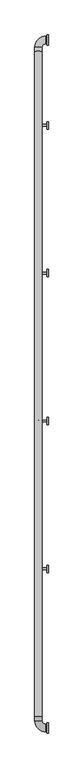
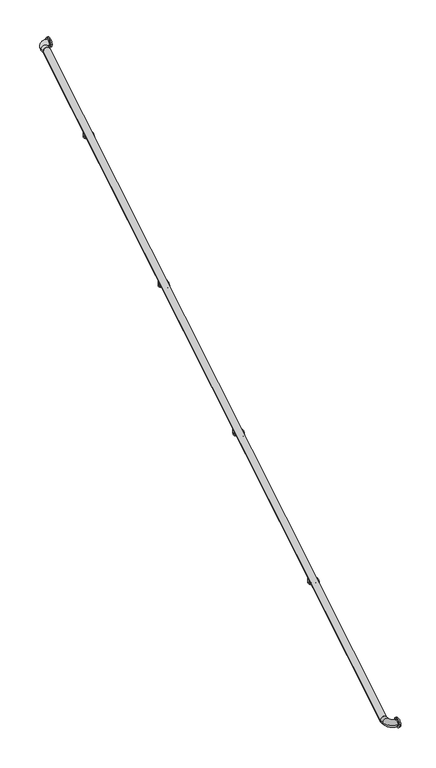
"""IFC4 building model written with IfcOpenShell, lengths in millimetres: railing geometry."""

from ifc_helpers import new_model, si_unit, point, frame, frame_2d, origin, place, context, project, spatial, circle_curve, ellipse_curve, trimmed, segment, composite_curve, outline, extrude, source, transform, mapped, element, save
from ifc_brep_helpers import plane_surface, cylinder_surface, revolved_surface, advanced_brep


def railing_debc8759(model_context):
    return source(origin(), model_context, "Body", "SolidModel", [
        advanced_brep(
        [(20407.2944438, 42249.3496945, 1051.653859), (20458.0944438, 42249.3496945, 1051.653859), (20407.2944438, 46749.3496945, 3771.653859), (20458.0944438, 46749.3496945, 3771.653859)],
        [
            (0, 1, ellipse_curve(frame((20432.6944438, 42249.3496945, 1051.653859), z_axis=(0.0, -1.0, 0.0), x_axis=(0.0, 0.0, -1.0)), 29.6794743, 25.4)),
            (1, 0, ellipse_curve(frame((20432.6944438, 42249.3496945, 1051.653859), z_axis=(0.0, -1.0, 0.0), x_axis=(0.0, 0.0, -1.0)), 29.6794743, 25.4)),
            (2, 3, ellipse_curve(frame((20432.6944438, 46749.3496945, 3771.653859), z_axis=(0.0, 1.0, 0.0), x_axis=(0.0, 0.0, -1.0)), 29.6794743, 25.4)),
            (3, 2, ellipse_curve(frame((20432.6944438, 46749.3496945, 3771.653859), z_axis=(0.0, 1.0, 0.0), x_axis=(0.0, 0.0, -1.0)), 29.6794743, 25.4)),
            (0, 2),
            (3, 1),
        ],
        [
            plane_surface(frame((20432.6944438, 42249.3496945, 1081.3333333), z_axis=(0.0, -1.0, 0.0), x_axis=(0.0, 0.0, 1.0))),
            plane_surface(frame((20432.6944438, 46749.3496945, 3801.3333333), z_axis=(0.0, 1.0, 0.0), x_axis=(0.0, 0.0, 1.0))),
            cylinder_surface(frame((20432.6944438, 42262.4888551, 1059.5957516), z_axis=(0.0, -0.8558103053667958, -0.5172897845772637), x_axis=(1.0, 0.0, 0.0)), 25.4),
        ],
        [
            (0, [[1, 2]]),
            (1, [[3, 4]]),
            (2, [[-1, 5, -4, 6]]),
            (2, [[-2, -6, -3, -5]]),
        ],
    ),
        extrude(outline(composite_curve([segment(trimmed(circle_curve(frame_2d((46249.3496945, 3363.7521624)), 25.4), [point((46274.7496945, 3363.7521624))], [point((46223.9496945, 3363.7521624))], False, "CARTESIAN"), True, "CONTINUOUS"), segment(trimmed(circle_curve(frame_2d((46249.3496945, 3363.7521624)), 25.4), [point((46223.9496945, 3363.7521624))], [point((46274.7496945, 3363.7521624))], False, "CARTESIAN"), True, "CONTINUOUS")], self_intersect=False)), frame((20490.1194438, 0.0, 0.0), z_axis=(1.0, 0.0, 0.0), x_axis=(0.0, 1.0, 0.0)), (0.0, 0.0, 1.0), 9.525),
        advanced_brep(
        [(20432.6444438, 46242.9996945, 3439.7521624), (20432.6444438, 46255.6996945, 3439.7521624), (20432.6444438, 46242.9996945, 3382.8021624), (20432.6444438, 46255.6996945, 3382.8021624), (20451.6944438, 46255.6996945, 3363.7521624), (20451.6944438, 46242.9996945, 3363.7521624), (20490.1194438, 46242.9996945, 3363.7521624), (20490.1194438, 46255.6996945, 3363.7521624)],
        [
            (0, 1, circle_curve(frame((20432.6444438, 46249.3496945, 3439.7521624), z_axis=(0.0, 0.0, 1.0), x_axis=(0.0, 1.0, 0.0)), 6.35)),
            (1, 0, circle_curve(frame((20432.6444438, 46249.3496945, 3439.7521624), z_axis=(0.0, 0.0, 1.0), x_axis=(0.0, 1.0, 0.0)), 6.35)),
            (0, 2),
            (2, 3, circle_curve(frame((20432.6444438, 46249.3496945, 3382.8021624), z_axis=(0.0, 0.0, 1.0), x_axis=(0.0, 1.0, 0.0)), 6.35)),
            (3, 1),
            (3, 2, circle_curve(frame((20432.6444438, 46249.3496945, 3382.8021624), z_axis=(0.0, 0.0, 1.0), x_axis=(0.0, 1.0, 0.0)), 6.35)),
            (4, 3, circle_curve(frame((20451.6944438, 46255.6996945, 3382.8021624), z_axis=(0.0, 1.0, 0.0), x_axis=(-1.0, 0.0, 0.0)), 19.05)),
            (2, 5, circle_curve(frame((20451.6944438, 46242.9996945, 3382.8021624), z_axis=(0.0, -1.0, 0.0), x_axis=(-1.0, 0.0, 0.0)), 19.05)),
            (5, 4, circle_curve(frame((20451.6944438, 46249.3496945, 3363.7521624), z_axis=(-1.0, 0.0, 0.0), x_axis=(0.0, 1.0, 0.0)), 6.35)),
            (4, 5, circle_curve(frame((20451.6944438, 46249.3496945, 3363.7521624), z_axis=(-1.0, 0.0, 0.0), x_axis=(0.0, 1.0, 0.0)), 6.35)),
            (6, 7, circle_curve(frame((20490.1194438, 46249.3496945, 3363.7521624), z_axis=(1.0, 0.0, 0.0), x_axis=(0.0, 1.0, 0.0)), 6.35)),
            (7, 6, circle_curve(frame((20490.1194438, 46249.3496945, 3363.7521624), z_axis=(1.0, 0.0, 0.0), x_axis=(0.0, 1.0, 0.0)), 6.35)),
            (5, 6),
            (7, 4),
        ],
        [
            plane_surface(frame((20432.6444438, 46255.6996945, 3439.7521624), z_axis=(0.0, 0.0, 1.0), x_axis=(1.0, 0.0, 0.0))),
            cylinder_surface(frame((20432.6444438, 46249.3496945, 3439.7521624), z_axis=(0.0, 0.0, 1.0), x_axis=(0.0, 1.0, 0.0)), 6.35),
            revolved_surface(trimmed(ellipse_curve(frame((20432.6444438, 46249.3496945, 3382.8021624), z_axis=(0.0, 0.0, 1.0), x_axis=(0.0, 1.0, 0.0)), 6.35, 6.35), [point((20432.6444438, 46242.9996945, 3382.8021624))], [point((20432.6444438, 46255.6996945, 3382.8021624))], True, "CARTESIAN"), (20451.6944438, 46249.3496945, 3382.8021624), (0.0, -1.0, 0.0)),
            revolved_surface(trimmed(ellipse_curve(frame((20432.6444438, 46249.3496945, 3382.8021624), z_axis=(0.0, 0.0, 1.0), x_axis=(0.0, 1.0, 0.0)), 6.35, 6.35), [point((20432.6444438, 46255.6996945, 3382.8021624))], [point((20432.6444438, 46242.9996945, 3382.8021624))], True, "CARTESIAN"), (20451.6944438, 46249.3496945, 3382.8021624), (0.0, -1.0, 0.0)),
            plane_surface(frame((20490.1194438, 46249.3496945, 3357.4021624), z_axis=(1.0, 0.0, 0.0), x_axis=(0.0, 1.0, 0.0))),
            cylinder_surface(frame((20451.6944438, 46249.3496945, 3363.7521624), z_axis=(-1.0, 0.0, 0.0), x_axis=(0.0, 1.0, 0.0)), 6.35),
        ],
        [
            (0, [[1, 2]]),
            (1, [[-1, 3, 4, 5]]),
            (1, [[-2, -5, 6, -3]]),
            (2, [[7, -4, 8, 9]]),
            (3, [[-8, -6, -7, 10]]),
            (4, [[11, 12]]),
            (5, [[-9, 13, -12, 14]]),
            (5, [[-10, -14, -11, -13]]),
        ],
    ),
        extrude(outline(composite_curve([segment(trimmed(circle_curve(frame_2d((45249.3496945, 2759.307718)), 25.4), [point((45274.7496945, 2759.307718))], [point((45223.9496945, 2759.307718))], False, "CARTESIAN"), True, "CONTINUOUS"), segment(trimmed(circle_curve(frame_2d((45249.3496945, 2759.307718)), 25.4), [point((45223.9496945, 2759.307718))], [point((45274.7496945, 2759.307718))], False, "CARTESIAN"), True, "CONTINUOUS")], self_intersect=False)), frame((20490.1194438, 0.0, 0.0), z_axis=(1.0, 0.0, 0.0), x_axis=(0.0, 1.0, 0.0)), (0.0, 0.0, 1.0), 9.525),
        advanced_brep(
        [(20432.6444438, 45242.9996945, 2835.307718), (20432.6444438, 45255.6996945, 2835.307718), (20432.6444438, 45242.9996945, 2778.357718), (20432.6444438, 45255.6996945, 2778.357718), (20451.6944438, 45255.6996945, 2759.307718), (20451.6944438, 45242.9996945, 2759.307718), (20490.1194438, 45242.9996945, 2759.307718), (20490.1194438, 45255.6996945, 2759.307718)],
        [
            (0, 1, circle_curve(frame((20432.6444438, 45249.3496945, 2835.307718), z_axis=(0.0, 0.0, 1.0), x_axis=(0.0, 1.0, 0.0)), 6.35)),
            (1, 0, circle_curve(frame((20432.6444438, 45249.3496945, 2835.307718), z_axis=(0.0, 0.0, 1.0), x_axis=(0.0, 1.0, 0.0)), 6.35)),
            (0, 2),
            (2, 3, circle_curve(frame((20432.6444438, 45249.3496945, 2778.357718), z_axis=(0.0, 0.0, 1.0), x_axis=(0.0, 1.0, 0.0)), 6.35)),
            (3, 1),
            (3, 2, circle_curve(frame((20432.6444438, 45249.3496945, 2778.357718), z_axis=(0.0, 0.0, 1.0), x_axis=(0.0, 1.0, 0.0)), 6.35)),
            (4, 3, circle_curve(frame((20451.6944438, 45255.6996945, 2778.357718), z_axis=(0.0, 1.0, 0.0), x_axis=(-1.0, 0.0, 0.0)), 19.05)),
            (2, 5, circle_curve(frame((20451.6944438, 45242.9996945, 2778.357718), z_axis=(0.0, -1.0, 0.0), x_axis=(-1.0, 0.0, 0.0)), 19.05)),
            (5, 4, circle_curve(frame((20451.6944438, 45249.3496945, 2759.307718), z_axis=(-1.0, 0.0, 0.0), x_axis=(0.0, 1.0, 0.0)), 6.35)),
            (4, 5, circle_curve(frame((20451.6944438, 45249.3496945, 2759.307718), z_axis=(-1.0, 0.0, 0.0), x_axis=(0.0, 1.0, 0.0)), 6.35)),
            (6, 7, circle_curve(frame((20490.1194438, 45249.3496945, 2759.307718), z_axis=(1.0, 0.0, 0.0), x_axis=(0.0, 1.0, 0.0)), 6.35)),
            (7, 6, circle_curve(frame((20490.1194438, 45249.3496945, 2759.307718), z_axis=(1.0, 0.0, 0.0), x_axis=(0.0, 1.0, 0.0)), 6.35)),
            (5, 6),
            (7, 4),
        ],
        [
            plane_surface(frame((20432.6444438, 45255.6996945, 2835.307718), z_axis=(0.0, 0.0, 1.0), x_axis=(1.0, 0.0, 0.0))),
            cylinder_surface(frame((20432.6444438, 45249.3496945, 2835.307718), z_axis=(0.0, 0.0, 1.0), x_axis=(0.0, 1.0, 0.0)), 6.35),
            revolved_surface(trimmed(ellipse_curve(frame((20432.6444438, 45249.3496945, 2778.357718), z_axis=(0.0, 0.0, 1.0), x_axis=(0.0, 1.0, 0.0)), 6.35, 6.35), [point((20432.6444438, 45242.9996945, 2778.357718))], [point((20432.6444438, 45255.6996945, 2778.357718))], True, "CARTESIAN"), (20451.6944438, 45249.3496945, 2778.357718), (0.0, -1.0, 0.0)),
            revolved_surface(trimmed(ellipse_curve(frame((20432.6444438, 45249.3496945, 2778.357718), z_axis=(0.0, 0.0, 1.0), x_axis=(0.0, 1.0, 0.0)), 6.35, 6.35), [point((20432.6444438, 45255.6996945, 2778.357718))], [point((20432.6444438, 45242.9996945, 2778.357718))], True, "CARTESIAN"), (20451.6944438, 45249.3496945, 2778.357718), (0.0, -1.0, 0.0)),
            plane_surface(frame((20490.1194438, 45249.3496945, 2752.957718), z_axis=(1.0, 0.0, 0.0), x_axis=(0.0, 1.0, 0.0))),
            cylinder_surface(frame((20451.6944438, 45249.3496945, 2759.307718), z_axis=(-1.0, 0.0, 0.0), x_axis=(0.0, 1.0, 0.0)), 6.35),
        ],
        [
            (0, [[1, 2]]),
            (1, [[-1, 3, 4, 5]]),
            (1, [[-2, -5, 6, -3]]),
            (2, [[7, -4, 8, 9]]),
            (3, [[-8, -6, -7, 10]]),
            (4, [[11, 12]]),
            (5, [[-9, 13, -12, 14]]),
            (5, [[-10, -14, -11, -13]]),
        ],
    ),
        extrude(outline(composite_curve([segment(trimmed(circle_curve(frame_2d((44249.3496945, 2154.8632735)), 25.4), [point((44274.7496945, 2154.8632735))], [point((44223.9496945, 2154.8632735))], False, "CARTESIAN"), True, "CONTINUOUS"), segment(trimmed(circle_curve(frame_2d((44249.3496945, 2154.8632735)), 25.4), [point((44223.9496945, 2154.8632735))], [point((44274.7496945, 2154.8632735))], False, "CARTESIAN"), True, "CONTINUOUS")], self_intersect=False)), frame((20490.1194438, 0.0, 0.0), z_axis=(1.0, 0.0, 0.0), x_axis=(0.0, 1.0, 0.0)), (0.0, 0.0, 1.0), 9.525),
        advanced_brep(
        [(20432.6444438, 44242.9996945, 2230.8632735), (20432.6444438, 44255.6996945, 2230.8632735), (20432.6444438, 44242.9996945, 2173.9132735), (20432.6444438, 44255.6996945, 2173.9132735), (20451.6944438, 44255.6996945, 2154.8632735), (20451.6944438, 44242.9996945, 2154.8632735), (20490.1194438, 44242.9996945, 2154.8632735), (20490.1194438, 44255.6996945, 2154.8632735)],
        [
            (0, 1, circle_curve(frame((20432.6444438, 44249.3496945, 2230.8632735), z_axis=(0.0, 0.0, 1.0), x_axis=(0.0, 1.0, 0.0)), 6.35)),
            (1, 0, circle_curve(frame((20432.6444438, 44249.3496945, 2230.8632735), z_axis=(0.0, 0.0, 1.0), x_axis=(0.0, 1.0, 0.0)), 6.35)),
            (0, 2),
            (2, 3, circle_curve(frame((20432.6444438, 44249.3496945, 2173.9132735), z_axis=(0.0, 0.0, 1.0), x_axis=(0.0, 1.0, 0.0)), 6.35)),
            (3, 1),
            (3, 2, circle_curve(frame((20432.6444438, 44249.3496945, 2173.9132735), z_axis=(0.0, 0.0, 1.0), x_axis=(0.0, 1.0, 0.0)), 6.35)),
            (4, 3, circle_curve(frame((20451.6944438, 44255.6996945, 2173.9132735), z_axis=(0.0, 1.0, 0.0), x_axis=(-1.0, 0.0, 0.0)), 19.05)),
            (2, 5, circle_curve(frame((20451.6944438, 44242.9996945, 2173.9132735), z_axis=(0.0, -1.0, 0.0), x_axis=(-1.0, 0.0, 0.0)), 19.05)),
            (5, 4, circle_curve(frame((20451.6944438, 44249.3496945, 2154.8632735), z_axis=(-1.0, 0.0, 0.0), x_axis=(0.0, 1.0, 0.0)), 6.35)),
            (4, 5, circle_curve(frame((20451.6944438, 44249.3496945, 2154.8632735), z_axis=(-1.0, 0.0, 0.0), x_axis=(0.0, 1.0, 0.0)), 6.35)),
            (6, 7, circle_curve(frame((20490.1194438, 44249.3496945, 2154.8632735), z_axis=(1.0, 0.0, 0.0), x_axis=(0.0, 1.0, 0.0)), 6.35)),
            (7, 6, circle_curve(frame((20490.1194438, 44249.3496945, 2154.8632735), z_axis=(1.0, 0.0, 0.0), x_axis=(0.0, 1.0, 0.0)), 6.35)),
            (5, 6),
            (7, 4),
        ],
        [
            plane_surface(frame((20432.6444438, 44255.6996945, 2230.8632735), z_axis=(0.0, 0.0, 1.0), x_axis=(1.0, 0.0, 0.0))),
            cylinder_surface(frame((20432.6444438, 44249.3496945, 2230.8632735), z_axis=(0.0, 0.0, 1.0), x_axis=(0.0, 1.0, 0.0)), 6.35),
            revolved_surface(trimmed(ellipse_curve(frame((20432.6444438, 44249.3496945, 2173.9132735), z_axis=(0.0, 0.0, 1.0), x_axis=(0.0, 1.0, 0.0)), 6.35, 6.35), [point((20432.6444438, 44242.9996945, 2173.9132735))], [point((20432.6444438, 44255.6996945, 2173.9132735))], True, "CARTESIAN"), (20451.6944438, 44249.3496945, 2173.9132735), (0.0, -1.0, 0.0)),
            revolved_surface(trimmed(ellipse_curve(frame((20432.6444438, 44249.3496945, 2173.9132735), z_axis=(0.0, 0.0, 1.0), x_axis=(0.0, 1.0, 0.0)), 6.35, 6.35), [point((20432.6444438, 44255.6996945, 2173.9132735))], [point((20432.6444438, 44242.9996945, 2173.9132735))], True, "CARTESIAN"), (20451.6944438, 44249.3496945, 2173.9132735), (0.0, -1.0, 0.0)),
            plane_surface(frame((20490.1194438, 44249.3496945, 2148.5132735), z_axis=(1.0, 0.0, 0.0), x_axis=(0.0, 1.0, 0.0))),
            cylinder_surface(frame((20451.6944438, 44249.3496945, 2154.8632735), z_axis=(-1.0, 0.0, 0.0), x_axis=(0.0, 1.0, 0.0)), 6.35),
        ],
        [
            (0, [[1, 2]]),
            (1, [[-1, 3, 4, 5]]),
            (1, [[-2, -5, 6, -3]]),
            (2, [[7, -4, 8, 9]]),
            (3, [[-8, -6, -7, 10]]),
            (4, [[11, 12]]),
            (5, [[-9, 13, -12, 14]]),
            (5, [[-10, -14, -11, -13]]),
        ],
    ),
        extrude(outline(composite_curve([segment(trimmed(circle_curve(frame_2d((43249.3496945, 1550.4188291)), 25.4), [point((43274.7496945, 1550.4188291))], [point((43223.9496945, 1550.4188291))], False, "CARTESIAN"), True, "CONTINUOUS"), segment(trimmed(circle_curve(frame_2d((43249.3496945, 1550.4188291)), 25.4), [point((43223.9496945, 1550.4188291))], [point((43274.7496945, 1550.4188291))], False, "CARTESIAN"), True, "CONTINUOUS")], self_intersect=False)), frame((20490.1194438, 0.0, 0.0), z_axis=(1.0, 0.0, 0.0), x_axis=(0.0, 1.0, 0.0)), (0.0, 0.0, 1.0), 9.525),
        advanced_brep(
        [(20432.6444438, 43242.9996945, 1626.4188291), (20432.6444438, 43255.6996945, 1626.4188291), (20432.6444438, 43242.9996945, 1569.4688291), (20432.6444438, 43255.6996945, 1569.4688291), (20451.6944438, 43255.6996945, 1550.4188291), (20451.6944438, 43242.9996945, 1550.4188291), (20490.1194438, 43242.9996945, 1550.4188291), (20490.1194438, 43255.6996945, 1550.4188291)],
        [
            (0, 1, circle_curve(frame((20432.6444438, 43249.3496945, 1626.4188291), z_axis=(0.0, 0.0, 1.0), x_axis=(0.0, 1.0, 0.0)), 6.35)),
            (1, 0, circle_curve(frame((20432.6444438, 43249.3496945, 1626.4188291), z_axis=(0.0, 0.0, 1.0), x_axis=(0.0, 1.0, 0.0)), 6.35)),
            (0, 2),
            (2, 3, circle_curve(frame((20432.6444438, 43249.3496945, 1569.4688291), z_axis=(0.0, 0.0, 1.0), x_axis=(0.0, 1.0, 0.0)), 6.35)),
            (3, 1),
            (3, 2, circle_curve(frame((20432.6444438, 43249.3496945, 1569.4688291), z_axis=(0.0, 0.0, 1.0), x_axis=(0.0, 1.0, 0.0)), 6.35)),
            (4, 3, circle_curve(frame((20451.6944438, 43255.6996945, 1569.4688291), z_axis=(0.0, 1.0, 0.0), x_axis=(-1.0, 0.0, 0.0)), 19.05)),
            (2, 5, circle_curve(frame((20451.6944438, 43242.9996945, 1569.4688291), z_axis=(0.0, -1.0, 0.0), x_axis=(-1.0, 0.0, 0.0)), 19.05)),
            (5, 4, circle_curve(frame((20451.6944438, 43249.3496945, 1550.4188291), z_axis=(-1.0, 0.0, 0.0), x_axis=(0.0, 1.0, 0.0)), 6.35)),
            (4, 5, circle_curve(frame((20451.6944438, 43249.3496945, 1550.4188291), z_axis=(-1.0, 0.0, 0.0), x_axis=(0.0, 1.0, 0.0)), 6.35)),
            (6, 7, circle_curve(frame((20490.1194438, 43249.3496945, 1550.4188291), z_axis=(1.0, 0.0, 0.0), x_axis=(0.0, 1.0, 0.0)), 6.35)),
            (7, 6, circle_curve(frame((20490.1194438, 43249.3496945, 1550.4188291), z_axis=(1.0, 0.0, 0.0), x_axis=(0.0, 1.0, 0.0)), 6.35)),
            (5, 6),
            (7, 4),
        ],
        [
            plane_surface(frame((20432.6444438, 43255.6996945, 1626.4188291), z_axis=(0.0, 0.0, 1.0), x_axis=(1.0, 0.0, 0.0))),
            cylinder_surface(frame((20432.6444438, 43249.3496945, 1626.4188291), z_axis=(0.0, 0.0, 1.0), x_axis=(0.0, 1.0, 0.0)), 6.35),
            revolved_surface(trimmed(ellipse_curve(frame((20432.6444438, 43249.3496945, 1569.4688291), z_axis=(0.0, 0.0, 1.0), x_axis=(0.0, 1.0, 0.0)), 6.35, 6.35), [point((20432.6444438, 43242.9996945, 1569.4688291))], [point((20432.6444438, 43255.6996945, 1569.4688291))], True, "CARTESIAN"), (20451.6944438, 43249.3496945, 1569.4688291), (0.0, -1.0, 0.0)),
            revolved_surface(trimmed(ellipse_curve(frame((20432.6444438, 43249.3496945, 1569.4688291), z_axis=(0.0, 0.0, 1.0), x_axis=(0.0, 1.0, 0.0)), 6.35, 6.35), [point((20432.6444438, 43255.6996945, 1569.4688291))], [point((20432.6444438, 43242.9996945, 1569.4688291))], True, "CARTESIAN"), (20451.6944438, 43249.3496945, 1569.4688291), (0.0, -1.0, 0.0)),
            plane_surface(frame((20490.1194438, 43249.3496945, 1544.0688291), z_axis=(1.0, 0.0, 0.0), x_axis=(0.0, 1.0, 0.0))),
            cylinder_surface(frame((20451.6944438, 43249.3496945, 1550.4188291), z_axis=(-1.0, 0.0, 0.0), x_axis=(0.0, 1.0, 0.0)), 6.35),
        ],
        [
            (0, [[1, 2]]),
            (1, [[-1, 3, 4, 5]]),
            (1, [[-2, -5, 6, -3]]),
            (2, [[7, -4, 8, 9]]),
            (3, [[-8, -6, -7, 10]]),
            (4, [[11, 12]]),
            (5, [[-9, 13, -12, 14]]),
            (5, [[-10, -14, -11, -13]]),
        ],
    ),
        extrude(outline(composite_curve([segment(trimmed(circle_curve(frame_2d((46825.3496945, 3776.0333333)), 35.4), [point((46860.7496945, 3776.0333333))], [point((46789.9496945, 3776.0333333))], False, "CARTESIAN"), True, "CONTINUOUS"), segment(trimmed(circle_curve(frame_2d((46825.3496945, 3776.0333333)), 35.4), [point((46789.9496945, 3776.0333333))], [point((46860.7496945, 3776.0333333))], False, "CARTESIAN"), True, "CONTINUOUS")], self_intersect=False)), frame((20490.1194438, 0.0, 0.0), z_axis=(1.0, 0.0, 0.0), x_axis=(0.0, 1.0, 0.0)), (0.0, 0.0, 1.0), 9.525),
        advanced_brep(
        [(20458.0444438, 46749.3496945, 3776.0333333), (20407.2444438, 46749.3496945, 3776.0333333), (20458.0444438, 46776.8496945, 3776.0333333), (20407.2444438, 46776.8496945, 3776.0333333), (20481.1444438, 46850.7496945, 3776.0333333), (20481.1444438, 46799.9496945, 3776.0333333), (20499.6444438, 46799.9496945, 3776.0333333), (20499.6444438, 46850.7496945, 3776.0333333)],
        [
            (0, 1, circle_curve(frame((20432.6444438, 46749.3496945, 3776.0333333), z_axis=(0.0, -1.0, 0.0), x_axis=(-1.0, 0.0, 0.0)), 25.4)),
            (1, 0, circle_curve(frame((20432.6444438, 46749.3496945, 3776.0333333), z_axis=(0.0, -1.0, 0.0), x_axis=(-1.0, 0.0, 0.0)), 25.4)),
            (0, 2),
            (2, 3, circle_curve(frame((20432.6444438, 46776.8496945, 3776.0333333), z_axis=(0.0, -1.0, 0.0), x_axis=(-1.0, 0.0, 0.0)), 25.4)),
            (3, 1),
            (3, 2, circle_curve(frame((20432.6444438, 46776.8496945, 3776.0333333), z_axis=(0.0, -1.0, 0.0), x_axis=(-1.0, 0.0, 0.0)), 25.4)),
            (4, 3, circle_curve(frame((20481.1444438, 46776.8496945, 3776.0333333), z_axis=(0.0, 0.0, 1.0), x_axis=(-1.0, 0.0, 0.0)), 73.9)),
            (2, 5, circle_curve(frame((20481.1444438, 46776.8496945, 3776.0333333), z_axis=(0.0, 0.0, -1.0), x_axis=(-1.0, 0.0, 0.0)), 23.1)),
            (5, 4, circle_curve(frame((20481.1444438, 46825.3496945, 3776.0333333), z_axis=(-1.0, 0.0, 0.0), x_axis=(0.0, 1.0, 0.0)), 25.4)),
            (4, 5, circle_curve(frame((20481.1444438, 46825.3496945, 3776.0333333), z_axis=(-1.0, 0.0, 0.0), x_axis=(0.0, 1.0, 0.0)), 25.4)),
            (6, 7, circle_curve(frame((20499.6444438, 46825.3496945, 3776.0333333), z_axis=(1.0, 0.0, 0.0), x_axis=(0.0, 1.0, 0.0)), 25.4)),
            (7, 6, circle_curve(frame((20499.6444438, 46825.3496945, 3776.0333333), z_axis=(1.0, 0.0, 0.0), x_axis=(0.0, 1.0, 0.0)), 25.4)),
            (5, 6),
            (7, 4),
        ],
        [
            plane_surface(frame((20432.6444438, 46749.3496945, 3776.0333333), z_axis=(0.0, -1.0, 0.0), x_axis=(0.0, 0.0, 1.0))),
            cylinder_surface(frame((20432.6444438, 46749.3496945, 3776.0333333), z_axis=(0.0, -1.0, 0.0), x_axis=(-1.0, 0.0, 0.0)), 25.4),
            revolved_surface(trimmed(ellipse_curve(frame((20432.6444438, 46776.8496945, 3776.0333333), z_axis=(0.0, -1.0, 0.0), x_axis=(-1.0, 0.0, 0.0)), 25.4, 25.4), [point((20458.0444438, 46776.8496945, 3776.0333333))], [point((20407.2444438, 46776.8496945, 3776.0333333))], True, "CARTESIAN"), (20481.1444438, 46776.8496945, 3776.0333333), (0.0, 0.0, -1.0)),
            revolved_surface(trimmed(ellipse_curve(frame((20432.6444438, 46776.8496945, 3776.0333333), z_axis=(0.0, -1.0, 0.0), x_axis=(-1.0, 0.0, 0.0)), 25.4, 25.4), [point((20407.2444438, 46776.8496945, 3776.0333333))], [point((20458.0444438, 46776.8496945, 3776.0333333))], True, "CARTESIAN"), (20481.1444438, 46776.8496945, 3776.0333333), (0.0, 0.0, -1.0)),
            plane_surface(frame((20499.6444438, 46825.3496945, 3776.0333333), z_axis=(1.0, 0.0, 0.0), x_axis=(0.0, 0.0, 1.0))),
            cylinder_surface(frame((20481.1444438, 46825.3496945, 3776.0333333), z_axis=(-1.0, 0.0, 0.0), x_axis=(0.0, 1.0, 0.0)), 25.4),
        ],
        [
            (0, [[1, 2]]),
            (1, [[-1, 3, 4, 5]]),
            (1, [[-2, -5, 6, -3]]),
            (2, [[7, -4, 8, 9]]),
            (3, [[-8, -6, -7, 10]]),
            (4, [[11, 12]]),
            (5, [[-9, 13, -12, 14]]),
            (5, [[-10, -14, -11, -13]]),
        ],
    ),
        extrude(outline(composite_curve([segment(trimmed(circle_curve(frame_2d((42173.3496945, 1056.0333333)), 35.4), [point((42208.7496945, 1056.0333333))], [point((42137.9496945, 1056.0333333))], False, "CARTESIAN"), True, "CONTINUOUS"), segment(trimmed(circle_curve(frame_2d((42173.3496945, 1056.0333333)), 35.4), [point((42137.9496945, 1056.0333333))], [point((42208.7496945, 1056.0333333))], False, "CARTESIAN"), True, "CONTINUOUS")], self_intersect=False)), frame((20490.1194438, 0.0, 0.0), z_axis=(1.0, 0.0, 0.0), x_axis=(0.0, 1.0, 0.0)), (0.0, 0.0, 1.0), 9.525),
        advanced_brep(
        [(20407.2444438, 42249.3496945, 1056.0333333), (20458.0444438, 42249.3496945, 1056.0333333), (20458.0444438, 42221.8496945, 1056.0333333), (20407.2444438, 42221.8496945, 1056.0333333), (20481.1444438, 42147.9496945, 1056.0333333), (20481.1444438, 42198.7496945, 1056.0333333), (20499.6444438, 42147.9496945, 1056.0333333), (20499.6444438, 42198.7496945, 1056.0333333)],
        [
            (0, 1, circle_curve(frame((20432.6444438, 42249.3496945, 1056.0333333), z_axis=(0.0, 1.0, 0.0), x_axis=(1.0, 0.0, 0.0)), 25.4)),
            (1, 0, circle_curve(frame((20432.6444438, 42249.3496945, 1056.0333333), z_axis=(0.0, 1.0, 0.0), x_axis=(1.0, 0.0, 0.0)), 25.4)),
            (1, 2),
            (2, 3, circle_curve(frame((20432.6444438, 42221.8496945, 1056.0333333), z_axis=(0.0, 1.0, 0.0), x_axis=(1.0, 0.0, 0.0)), 25.4)),
            (3, 0),
            (3, 2, circle_curve(frame((20432.6444438, 42221.8496945, 1056.0333333), z_axis=(0.0, 1.0, 0.0), x_axis=(1.0, 0.0, 0.0)), 25.4)),
            (4, 3, circle_curve(frame((20481.1444438, 42221.8496945, 1056.0333333), z_axis=(0.0, 0.0, -1.0), x_axis=(-1.0, 0.0, 0.0)), 73.9)),
            (2, 5, circle_curve(frame((20481.1444438, 42221.8496945, 1056.0333333), z_axis=(0.0, 0.0, 1.0), x_axis=(-1.0, 0.0, 0.0)), 23.1)),
            (5, 4, circle_curve(frame((20481.1444438, 42173.3496945, 1056.0333333), z_axis=(-1.0, 0.0, 0.0), x_axis=(0.0, 1.0, 0.0)), 25.4)),
            (4, 5, circle_curve(frame((20481.1444438, 42173.3496945, 1056.0333333), z_axis=(-1.0, 0.0, 0.0), x_axis=(0.0, 1.0, 0.0)), 25.4)),
            (6, 7, circle_curve(frame((20499.6444438, 42173.3496945, 1056.0333333), z_axis=(1.0, 0.0, 0.0), x_axis=(0.0, 1.0, 0.0)), 25.4)),
            (7, 6, circle_curve(frame((20499.6444438, 42173.3496945, 1056.0333333), z_axis=(1.0, 0.0, 0.0), x_axis=(0.0, 1.0, 0.0)), 25.4)),
            (5, 7),
            (6, 4),
        ],
        [
            plane_surface(frame((20432.6444438, 42249.3496945, 1056.0333333), z_axis=(0.0, 1.0, 0.0), x_axis=(0.0, 0.0, 1.0))),
            cylinder_surface(frame((20432.6444438, 42249.3496945, 1056.0333333), z_axis=(0.0, 1.0, 0.0), x_axis=(1.0, 0.0, 0.0)), 25.4),
            revolved_surface(trimmed(ellipse_curve(frame((20432.6444438, 42221.8496945, 1056.0333333), z_axis=(0.0, 1.0, 0.0), x_axis=(1.0, 0.0, 0.0)), 25.4, 25.4), [point((20458.0444438, 42221.8496945, 1056.0333333))], [point((20407.2444438, 42221.8496945, 1056.0333333))], True, "CARTESIAN"), (20481.1444438, 42221.8496945, 1056.0333333), (0.0, 0.0, 1.0)),
            revolved_surface(trimmed(ellipse_curve(frame((20432.6444438, 42221.8496945, 1056.0333333), z_axis=(0.0, 1.0, 0.0), x_axis=(1.0, 0.0, 0.0)), 25.4, 25.4), [point((20407.2444438, 42221.8496945, 1056.0333333))], [point((20458.0444438, 42221.8496945, 1056.0333333))], True, "CARTESIAN"), (20481.1444438, 42221.8496945, 1056.0333333), (0.0, 0.0, 1.0)),
            plane_surface(frame((20499.6444438, 42173.3496945, 1056.0333333), z_axis=(1.0, 0.0, 0.0), x_axis=(0.0, 0.0, 1.0))),
            cylinder_surface(frame((20481.1444438, 42173.3496945, 1056.0333333), z_axis=(-1.0, 0.0, 0.0), x_axis=(0.0, 1.0, 0.0)), 25.4),
        ],
        [
            (0, [[1, 2]]),
            (1, [[-2, 3, 4, 5]]),
            (1, [[-1, -5, 6, -3]]),
            (2, [[7, -4, 8, 9]]),
            (3, [[-8, -6, -7, 10]]),
            (4, [[11, 12]]),
            (5, [[-9, 13, -11, 14]]),
            (5, [[-10, -14, -12, -13]]),
        ],
    ),
    ])


if __name__ == "__main__":
    model = new_model("IFC4")
    model_context = context("Model", 3, world=origin())
    ifc_project = project(units=[si_unit("LENGTHUNIT", "METRE", prefix="MILLI")], contexts=[model_context])
    site = spatial("IfcSite", under=ifc_project)
    building = spatial("IfcBuilding", under=site)
    placement = place(None, origin())
    railing_shape = railing_debc8759(model_context)
    element("IfcRailing", 1, at=placement, inside=building, context=model_context, shape_type="MappedRepresentation", body=[
        mapped(railing_shape, transform((0.0, 0.0, 0.0), x_axis=(1.0, 0.0, 0.0), y_axis=(0.0, 1.0, 0.0), z_axis=(0.0, 0.0, 1.0))),
    ])
    save(model, "model.ifc")

# Revit data of these elements
# Element 1 (IfcRailing)
#   Materials on its faces: "Ferro - Pintura Esmalte"
# Materials
#   "Ferro - Pintura Esmalte": class "Pintura", colour RGB 255 255 255, transparency 0, Cost = 0
